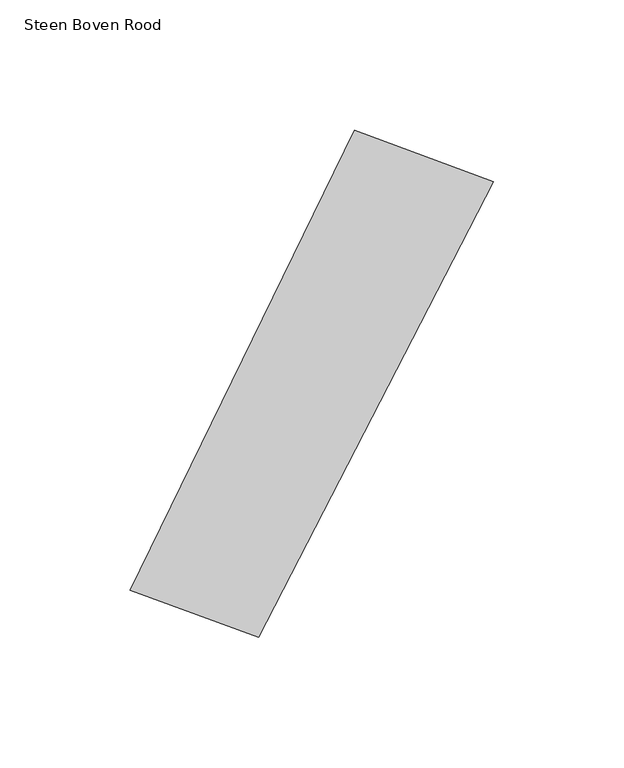
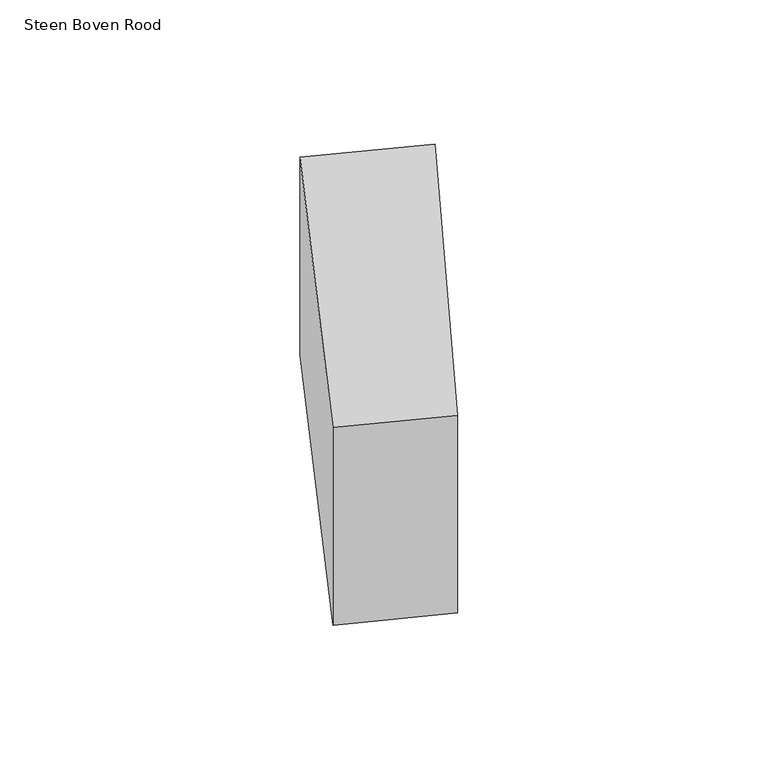
"""IFC4 building model written with IfcOpenShell, lengths in millimetres: proxy geometry, 00_GMA_steen_versie_4 : Steen Boven Rood."""

from ifc_helpers import new_model, si_unit, origin, origin_with_axes, place, context, project, spatial, polyline, outline, extrude, source, transform, mapped, element, save


def steen_boven_rood_39178d75(model_context):
    return source(origin(), model_context, "Body", "SweptSolid", [
        extrude(outline(polyline([(147.0451075, 159.8682893), (56.9755351, -14.7591453), (7.903048, 3.4193083), (93.9034048, 179.5423978), (147.0451075, 159.8682893)])), origin_with_axes(), (0.0, 0.0, 1.0), 100.0),
    ])


if __name__ == "__main__":
    model = new_model("IFC4")
    model_context = context("Model", 3, world=origin())
    ifc_project = project(units=[si_unit("LENGTHUNIT", "METRE", prefix="MILLI")], contexts=[model_context])
    site = spatial("IfcSite", under=ifc_project)
    building = spatial("IfcBuilding", under=site)
    placement = place(None, origin())
    steen_boven_rood_shape = steen_boven_rood_39178d75(model_context)
    element("IfcBuildingElementProxy", 1, Name="00_GMA_steen_versie_4 : Steen Boven Rood", ObjectType="00_GMA_steen_versie_4 : Steen Boven Rood", at=placement, inside=building, context=model_context, shape_type="MappedRepresentation", body=[
        mapped(steen_boven_rood_shape, transform((0.0, 0.0, 0.0), x_axis=(1.0, 0.0, 0.0), y_axis=(0.0, 1.0, 0.0), z_axis=(0.0, 0.0, 1.0))),
    ])
    save(model, "model.ifc")

# Revit data of these elements
# Type "00_GMA_steen_versie_4 : Steen Boven Rood"
#   StootVoegHalfBoven [instance default] = 5 mm
#   StootVoegHalf [instance default] = 5 mm
#   StootVoegBreedteOnder = 10 mm
#   StootVoegBreedteBoven = 10 mm
#   Steendikte = 100 mm
#   LintVoegOnderHalf = 5 mm
#   LintVoegOnder = 10 mm
#   LintVoegBovenHalf = 0 mm
#   LintVoegBoven = 0 mm
#   materiaal = 21_steen_rood
#   MateriaalVoeg = none
#   Default Elevation = 0
# Element 1 (IfcBuildingElementProxy, "00_GMA_steen_versie_4 : Steen Boven Rood")
#   Materials on its faces: "21_steen_rood"
# Materials
#   "21_steen_rood": class "Unassigned", colour RGB 213 111 43, transparency 0, Cost = 0
